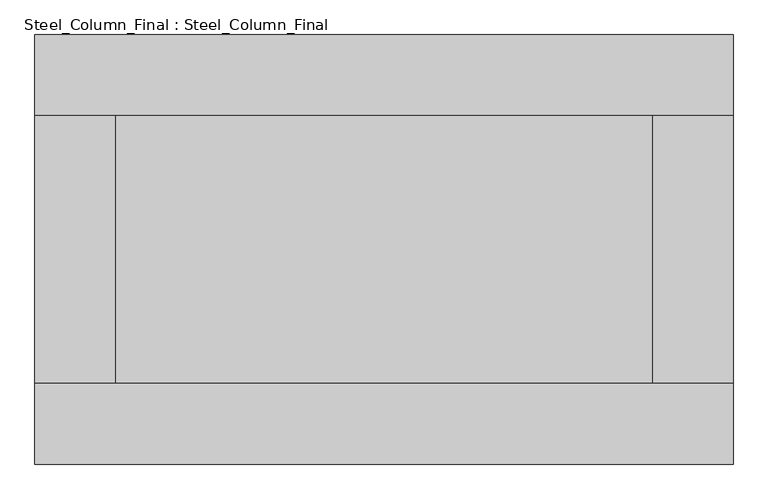
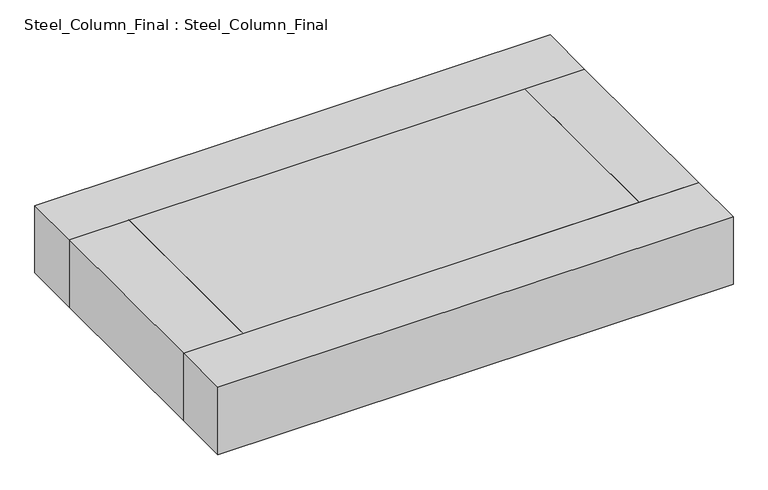
"""IFC4 building model written with IfcOpenShell, lengths in millimetres: proxy geometry, Steel_Column_Final : Steel_Column_Final."""

from ifc_helpers import new_model, si_unit, frame, origin, place, context, project, spatial, polyline, outline, extrude, source, transform, mapped, element, save


def steel_column_final_steel_column_final_7508d8fd(model_context):
    return source(origin(), model_context, "Body", "SweptSolid", [
        extrude(outline(polyline([(6500.0, 2500.0), (-6500.0, 2500.0), (-6500.0, 4000.0), (6500.0, 4000.0), (6500.0, 2500.0)])), frame((0.0, 0.0, 55500.0), z_axis=(0.0, 0.0, 1.0), x_axis=(1.0, 0.0, 0.0)), (0.0, 0.0, 1.0), 1800.0),
        extrude(outline(polyline([(-6500.0, -2500.0), (6500.0, -2500.0), (6500.0, -4000.0), (-6500.0, -4000.0), (-6500.0, -2500.0)])), frame((0.0, 0.0, 55500.0), z_axis=(0.0, 0.0, 1.0), x_axis=(1.0, 0.0, 0.0)), (0.0, 0.0, 1.0), 1800.0),
        extrude(outline(polyline([(5000.0, -2500.0), (5000.0, 2500.0), (6500.0, 2500.0), (6500.0, -2500.0), (5000.0, -2500.0)])), frame((0.0, 0.0, 55500.0), z_axis=(0.0, 0.0, 1.0), x_axis=(1.0, 0.0, 0.0)), (0.0, 0.0, 1.0), 1800.0),
        extrude(outline(polyline([(-5000.0, 2500.0), (-5000.0, -2500.0), (-6500.0, -2500.0), (-6500.0, 2500.0), (-5000.0, 2500.0)])), frame((0.0, 0.0, 55500.0), z_axis=(0.0, 0.0, 1.0), x_axis=(1.0, 0.0, 0.0)), (0.0, 0.0, 1.0), 1800.0),
        extrude(outline(polyline([(-5000.0, -2500.0), (-5000.0, 2500.0), (5000.0, 2500.0), (5000.0, -2500.0), (-5000.0, -2500.0)])), frame((0.0, 0.0, 55500.0), z_axis=(0.0, 0.0, 1.0), x_axis=(1.0, 0.0, 0.0)), (0.0, 0.0, 1.0), 1800.0),
    ])


if __name__ == "__main__":
    model = new_model("IFC4")
    model_context = context("Model", 3, world=origin())
    ifc_project = project(units=[si_unit("LENGTHUNIT", "METRE", prefix="MILLI")], contexts=[model_context])
    site = spatial("IfcSite", under=ifc_project)
    building = spatial("IfcBuilding", under=site)
    placement = place(None, origin())
    steel_column_final_steel_column_final_shape = steel_column_final_steel_column_final_7508d8fd(model_context)
    element("IfcBuildingElementProxy", 1, Name="Steel_Column_Final : Steel_Column_Final", ObjectType="Steel_Column_Final : Steel_Column_Final", at=placement, inside=building, context=model_context, shape_type="MappedRepresentation", body=[
        mapped(steel_column_final_steel_column_final_shape, transform((0.0, 0.0, 0.0), x_axis=(1.0, 0.0, 0.0), y_axis=(0.0, 1.0, 0.0), z_axis=(0.0, 0.0, 1.0))),
    ])
    save(model, "model.ifc")

# Revit data of these elements
# Type "Steel_Column_Final : Steel_Column_Final"
#   Top Width [instance default] = 5000 mm
#   Top Length = 10000 mm
#   Length = 21000 mm
#   Height [instance default] = 50000 mm
#   Bottom Width [instance default] = 5000 mm
#   Default Elevation = 0
# Element 1 (IfcBuildingElementProxy, "Steel_Column_Final : Steel_Column_Final")
#   Height = 55500 mm
